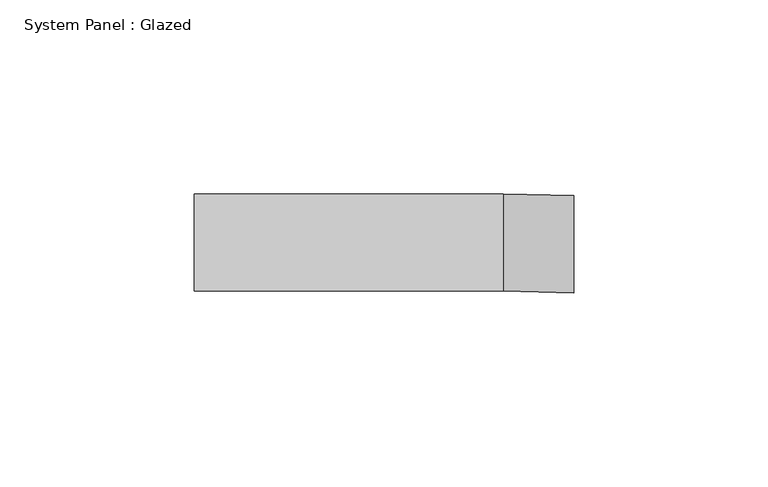
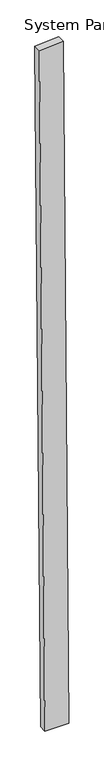
"""IFC4 building model written with IfcOpenShell, lengths in millimetres: plate geometry, System Panel : Glazed."""

from ifc_helpers import new_model, si_unit, frame, origin, place, context, project, spatial, polyline, outline, extrude, source, transform, mapped, element, save


def system_panel_glazed_4dd55457(model_context):
    return source(origin(), model_context, "Body", "SweptSolid", [
        extrude(outline(polyline([(0.0, -30.1852095), (0.0, 48.8417218), (2397.9897252, 30.6680018), (2392.2849165, -48.8417218), (0.0, -30.1852095)])), frame((0.0, -49.5, 0.0), z_axis=(0.0, 1.0, 0.0), x_axis=(0.0, 0.0, 1.0)), (0.0, 0.0, 1.0), 25.0),
    ])


if __name__ == "__main__":
    model = new_model("IFC4")
    model_context = context("Model", 3, world=origin())
    ifc_project = project(units=[si_unit("LENGTHUNIT", "METRE", prefix="MILLI")], contexts=[model_context])
    site = spatial("IfcSite", under=ifc_project)
    building = spatial("IfcBuilding", under=site)
    placement = place(None, origin())
    system_panel_glazed_shape = system_panel_glazed_4dd55457(model_context)
    element("IfcPlate", 1, ObjectType="System Panel : Glazed", at=placement, inside=building, context=model_context, shape_type="MappedRepresentation", body=[
        mapped(system_panel_glazed_shape, transform((0.0, 0.0, 0.0), x_axis=(1.0, 0.0, 0.0), y_axis=(0.0, 1.0, 0.0), z_axis=(0.0, 0.0, 1.0))),
    ])
    save(model, "model.ifc")

# Revit data of these elements
# Element 1 (IfcPlate, "System Panel : Glazed")
#   Materials on its faces: "Glass, Clear Glazing"
# Materials
#   "Glass, Clear Glazing": class "Glass", colour RGB 247 249 248, transparency 0.85, Description = "Clear glazing", Cost = 0
